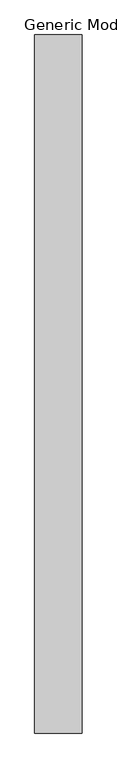
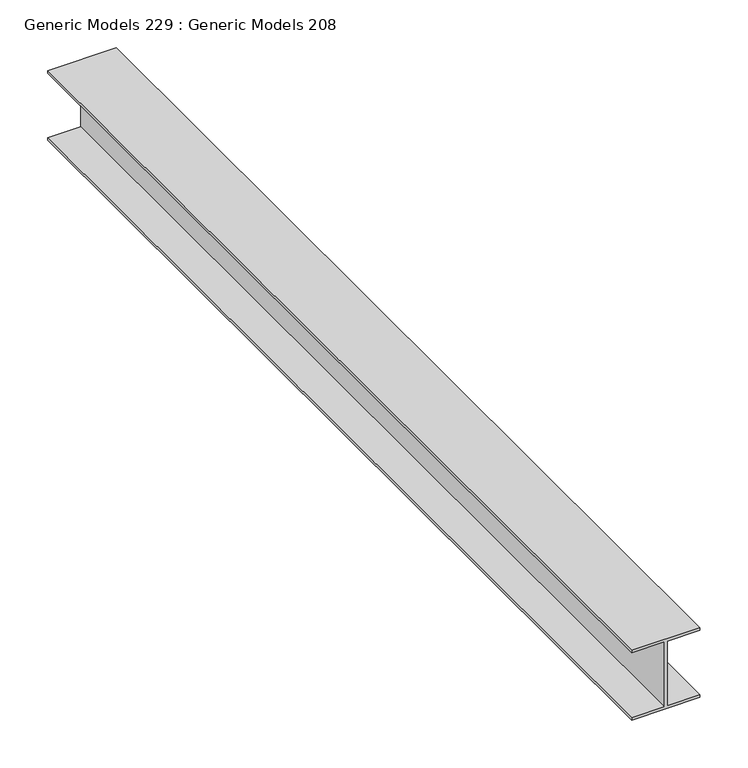
"""IFC4 building model written with IfcOpenShell, lengths in millimetres: proxy geometry, Generic Models 229 : Generic Models 208."""

from ifc_helpers import new_model, si_unit, frame, origin, place, context, project, spatial, polyline, outline, extrude, source, transform, mapped, element, save


def generic_models_229_generic_models_208_12bc7626(model_context):
    return source(origin(), model_context, "Body", "SweptSolid", [
        extrude(outline(polyline([(2257.425, 54420.2704676), (2257.425, 54459.9579676), (2260.6, 54459.9579676), (2260.6, 54377.4079676), (2257.425, 54377.4079676), (2257.425, 54417.0954676), (2174.875, 54417.0954676), (2174.875, 54377.4079676), (2171.7, 54377.4079676), (2171.7, 54459.9579676), (2174.875, 54459.9579676), (2174.875, 54420.2704676), (2257.425, 54420.2704676)])), frame((0.0, -228.7033818, 0.0), z_axis=(0.0, 1.0, 0.0), x_axis=(0.0, 0.0, 1.0)), (0.0, 0.0, 1.0), 1219.2),
    ])


if __name__ == "__main__":
    model = new_model("IFC4")
    model_context = context("Model", 3, world=origin())
    ifc_project = project(units=[si_unit("LENGTHUNIT", "METRE", prefix="MILLI")], contexts=[model_context])
    site = spatial("IfcSite", under=ifc_project)
    building = spatial("IfcBuilding", under=site)
    placement = place(None, origin())
    generic_models_229_generic_models_208_shape = generic_models_229_generic_models_208_12bc7626(model_context)
    element("IfcBuildingElementProxy", 1, Name="Generic Models 229 : Generic Models 208", ObjectType="Generic Models 229 : Generic Models 208", at=placement, inside=building, context=model_context, shape_type="MappedRepresentation", body=[
        mapped(generic_models_229_generic_models_208_shape, transform((0.0, 0.0, 0.0), x_axis=(1.0, 0.0, 0.0), y_axis=(0.0, 1.0, 0.0), z_axis=(0.0, 0.0, 1.0))),
    ])
    save(model, "model.ifc")
